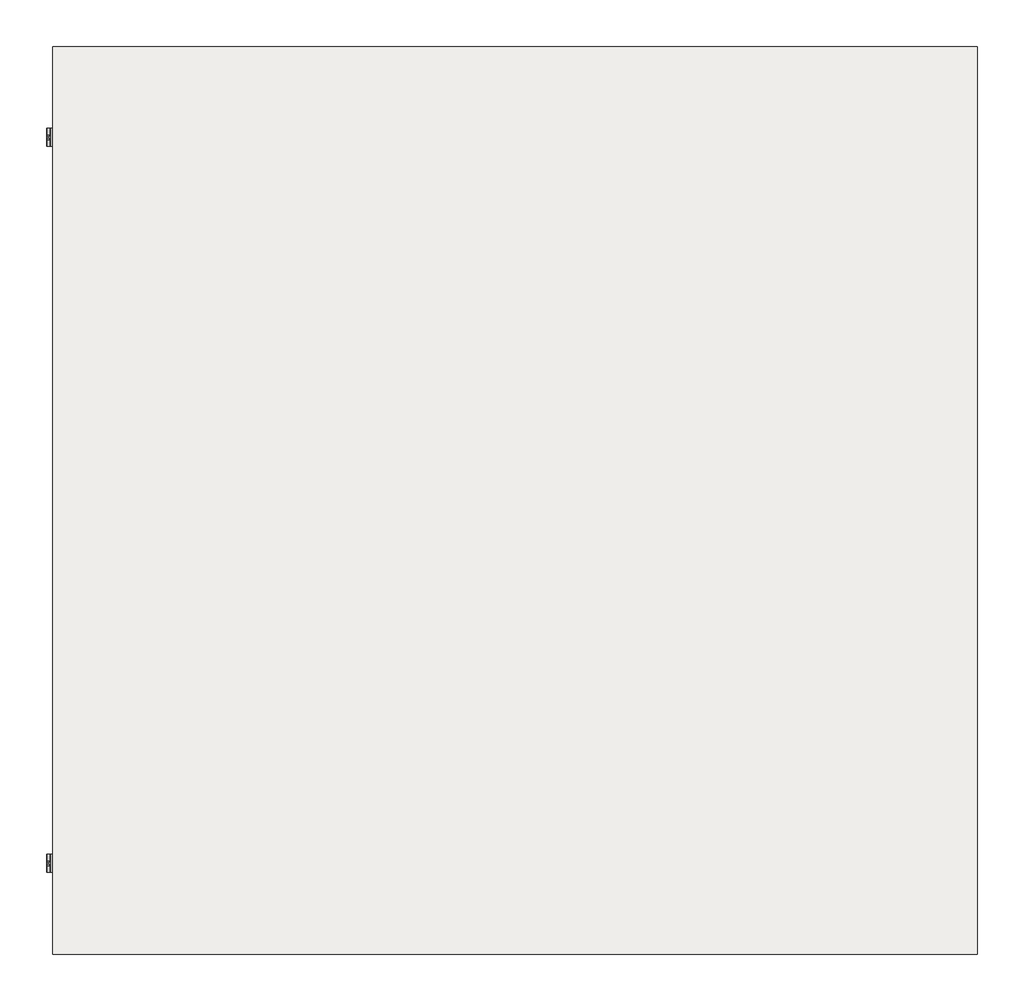
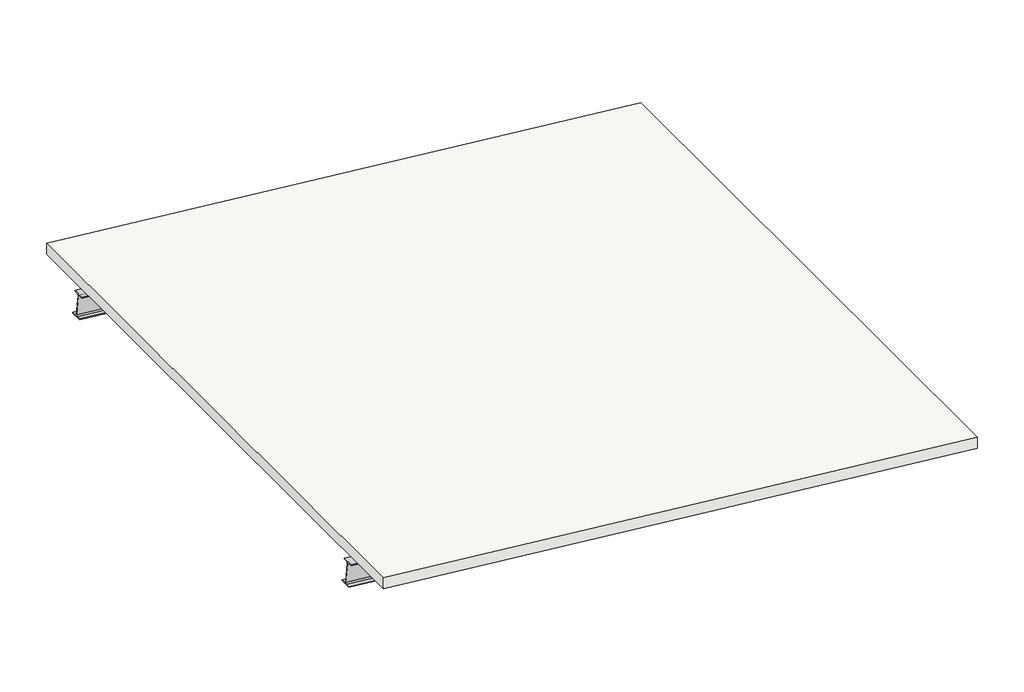
# One storey: 4 beams, 1 roof.
"""IFC4 building model written with IfcOpenShell, lengths in millimetres."""

import ifcopenshell
import ifcopenshell.guid

model = None  # the IFC model being written
_history = None  # IfcOwnerHistory: only IFC2X3 demands one
_inside = {}  # id of a spatial element -> (the spatial element, [elements in it])
_under = {}  # id of a project, library or spatial element -> (it, [spatial elements below it])
_declared = {}  # id of a project -> (the project, [libraries it declares])
_typed = {}  # id of a type object -> (the type object, [elements of that type])
_made_of = {}  # id of a material, layer set ... -> (it, [elements and type objects made of it])


def new_model(schema):
    """Start an empty IFC model of exactly this schema.

    Asked for "IFC4X3", IfcOpenShell would pick the latest addendum, in which some entities
    have other attributes; the version numbers below select the first issue.
    IFC2X3 requires an IfcOwnerHistory on every rooted entity: one is made here for all.
    """
    global model, _history
    if schema == "IFC4X3":
        model = ifcopenshell.file(schema_version=(4, 3, 0, 0))
    else:
        model = ifcopenshell.file(schema=schema)
    _inside.clear()
    _under.clear()
    _declared.clear()
    _typed.clear()
    _made_of.clear()
    _history = None
    if model.schema == "IFC2X3":
        org = make("IfcOrganization", Name="unknown")
        user = make(
            "IfcPersonAndOrganization",
            ThePerson=make("IfcPerson", FamilyName="unknown"),
            TheOrganization=org,
        )
        app = make(
            "IfcApplication",
            ApplicationDeveloper=org,
            Version="unknown",
            ApplicationFullName="unknown",
            ApplicationIdentifier="unknown",
        )
        _history = make(
            "IfcOwnerHistory",
            OwningUser=user,
            OwningApplication=app,
            ChangeAction="ADDED",
            CreationDate=0,
        )
    return model


def make(cls, **values):
    """One entity of the class cls with the attributes given. An attribute that is None is left unset."""
    return model.create_entity(
        cls, **{name: value for name, value in values.items() if value is not None}
    )


def rooted(cls, **values):
    """An entity with a GlobalId (a new one), such as an element, a storey or a relation."""
    return make(cls, GlobalId=ifcopenshell.guid.new(), OwnerHistory=_history, **values)


def si_unit(unit_type, name, prefix=None):
    """IfcSIUnit, for example si_unit("LENGTHUNIT", "METRE", prefix="MILLI")."""
    return make("IfcSIUnit", UnitType=unit_type, Prefix=prefix, Name=name)


def assignment(units):
    """IfcUnitAssignment: the units of a project."""
    return None if units is None else make("IfcUnitAssignment", Units=units)


def point(xyz):
    """IfcCartesianPoint."""
    return None if xyz is None else make("IfcCartesianPoint", Coordinates=xyz)


def direction(xyz):
    """IfcDirection."""
    return None if xyz is None else make("IfcDirection", DirectionRatios=xyz)


def frame(location, z_axis=None, x_axis=None):
    """IfcAxis2Placement3D, a coordinate frame: its origin and axes. An axis left out is left unset."""
    return make(
        "IfcAxis2Placement3D",
        Location=point(location),
        Axis=direction(z_axis),
        RefDirection=direction(x_axis),
    )


def frame_2d(location, x_axis=None):
    """IfcAxis2Placement2D, a coordinate frame in the plane: its origin and x axis."""
    return make(
        "IfcAxis2Placement2D", Location=point(location), RefDirection=direction(x_axis)
    )


def origin():
    """The frame at (0, 0, 0) with its axes left unset."""
    return frame((0.0, 0.0, 0.0))


def place(relative_to, where):
    """IfcLocalPlacement: puts the frame where relative to a parent placement (None: the world)."""
    return make(
        "IfcLocalPlacement", PlacementRelTo=relative_to, RelativePlacement=where
    )


def context(
    kind, dimensions, precision=None, world=None, true_north=None, identifier=None
):
    """IfcGeometricRepresentationContext, for example the 3D "Model" context."""
    return make(
        "IfcGeometricRepresentationContext",
        ContextIdentifier=identifier,
        ContextType=kind,
        CoordinateSpaceDimension=dimensions,
        Precision=precision,
        WorldCoordinateSystem=world,
        TrueNorth=true_north,
    )


def project(units=None, contexts=None):
    """IfcProject with its units and contexts."""
    return rooted(
        "IfcProject",
        Name="project",
        RepresentationContexts=contexts,
        UnitsInContext=assignment(units),
    )


def spatial(cls, under=None, at=None, **own):
    """A site, building, storey or space (cls), placed at a placement, below another one or the project."""
    s = rooted(cls, ObjectPlacement=at, **own)
    if under is not None:
        _under.setdefault(under.id(), (under, []))[1].append(s)
    return s


def polyline(points):
    """IfcPolyline through the points."""
    return make("IfcPolyline", Points=[point(p) for p in points])


def circle_curve(where, radius):
    """IfcCircle in the frame where."""
    return make("IfcCircle", Position=where, Radius=radius)


def trimmed(basis, trim1, trim2, sense, master):
    """IfcTrimmedCurve: the piece of a basis curve between two trims."""
    return make(
        "IfcTrimmedCurve",
        BasisCurve=basis,
        Trim1=trim1,
        Trim2=trim2,
        SenseAgreement=sense,
        MasterRepresentation=master,
    )


def segment(curve, same_sense, transition):
    """IfcCompositeCurveSegment."""
    return make(
        "IfcCompositeCurveSegment",
        Transition=transition,
        SameSense=same_sense,
        ParentCurve=curve,
    )


def composite_curve(segments, self_intersect=None):
    """IfcCompositeCurve: segments joined end to end."""
    return make("IfcCompositeCurve", Segments=segments, SelfIntersect=self_intersect)


def outline(outer, holes=None, kind="AREA"):
    """IfcArbitraryClosedProfileDef: a profile drawn as a closed curve; with holes, ...WithVoids."""
    if holes is None:
        return make("IfcArbitraryClosedProfileDef", ProfileType=kind, OuterCurve=outer)
    return make(
        "IfcArbitraryProfileDefWithVoids",
        ProfileType=kind,
        OuterCurve=outer,
        InnerCurves=holes,
    )


def extrude(swept, where, along, depth):
    """IfcExtrudedAreaSolid: the profile swept, set in the frame where, extruded along a direction by depth."""
    return make(
        "IfcExtrudedAreaSolid",
        SweptArea=swept,
        Position=where,
        ExtrudedDirection=direction(along),
        Depth=depth,
    )


def shape(context_of_items, identifier, shape_type, items):
    """IfcShapeRepresentation: the items that make up one representation, for example the "Body"."""
    return make(
        "IfcShapeRepresentation",
        ContextOfItems=context_of_items,
        RepresentationIdentifier=identifier,
        RepresentationType=shape_type,
        Items=items,
    )


def source(mapping_origin, context_of_items, identifier, shape_type, items):
    """IfcRepresentationMap: a shape defined once, which mapped items show again and again."""
    return make(
        "IfcRepresentationMap",
        MappingOrigin=mapping_origin,
        MappedRepresentation=shape(context_of_items, identifier, shape_type, items),
    )


def transform(
    local_origin,
    x_axis=None,
    y_axis=None,
    z_axis=None,
    scale=None,
    scale2=None,
    scale3=None,
    uniform=True,
):
    """IfcCartesianTransformationOperator3D, or its non-uniform kind. x_axis, y_axis, z_axis: its Axis1, 2, 3."""
    if uniform:
        return make(
            "IfcCartesianTransformationOperator3D",
            Axis1=direction(x_axis),
            Axis2=direction(y_axis),
            LocalOrigin=point(local_origin),
            Scale=scale,
            Axis3=direction(z_axis),
        )
    return make(
        "IfcCartesianTransformationOperator3DnonUniform",
        Axis1=direction(x_axis),
        Axis2=direction(y_axis),
        LocalOrigin=point(local_origin),
        Scale=scale,
        Axis3=direction(z_axis),
        Scale2=scale2,
        Scale3=scale3,
    )


def mapped(mapping_source, mapping_target):
    """IfcMappedItem: shows the shape of a source again, moved by a transform."""
    return make(
        "IfcMappedItem", MappingSource=mapping_source, MappingTarget=mapping_target
    )


def made_of(thing, what):
    """Note that an element or type object is made of a material, layer set ...; save() writes the relation."""
    if what is not None:
        _made_of.setdefault(what.id(), (what, []))[1].append(thing)
    return thing


def element(
    cls,
    number,
    at=None,
    inside=None,
    cuts=None,
    type_object=None,
    material=None,
    context=None,
    identifier="Body",
    shape_type=None,
    held_by="IfcProductDefinitionShape",
    body=None,
    shapes=None,
    **own,
):
    """One element of the class cls, such as IfcWall. Its Tag is "e" and its number.

    at: its placement. inside: the storey or other place that contains it. cuts: it is an
    opening in that element (IfcRelVoidsElement). A single representation is given by context,
    identifier, shape_type and body (its items); several are given by shapes. held_by: the class
    of the entity that holds the representations. save() writes the other relations.
    """
    e = rooted(cls, Tag="e%d" % number, ObjectPlacement=at, **own)
    if body is not None:
        shapes = [shape(context, identifier, shape_type, body)]
    if shapes is not None:
        e.Representation = make(held_by, Representations=shapes)
    if inside is not None:
        _inside.setdefault(inside.id(), (inside, []))[1].append(e)
    if cuts is not None:
        rooted(
            "IfcRelVoidsElement", RelatingBuildingElement=cuts, RelatedOpeningElement=e
        )
    if type_object is not None:
        _typed.setdefault(type_object.id(), (type_object, []))[1].append(e)
    return made_of(e, material)


def aggregate(whole, parts):
    """IfcRelAggregates: a whole, such as a stair, and the parts it consists of."""
    return rooted("IfcRelAggregates", RelatingObject=whole, RelatedObjects=parts)


def save(model, path):
    """Write the relations noted so far, then the file.

    IfcRelAggregates (storeys below a building ...), IfcRelContainedInSpatialStructure (elements
    in a storey), IfcRelDefinesByType, IfcRelAssociatesMaterial and IfcRelDeclares: one each for
    every whole, place, type object, material and project.
    """
    for whole, parts in _under.values():
        aggregate(whole, parts)
    for where, things in _inside.values():
        rooted(
            "IfcRelContainedInSpatialStructure",
            RelatedElements=things,
            RelatingStructure=where,
        )
    for kind, things in _typed.values():
        rooted("IfcRelDefinesByType", RelatedObjects=things, RelatingType=kind)
    for what, things in _made_of.values():
        rooted("IfcRelAssociatesMaterial", RelatedObjects=things, RelatingMaterial=what)
    for by, libraries in _declared.values():
        rooted("IfcRelDeclares", RelatingContext=by, RelatedDefinitions=libraries)
    model.write(path)


def beam_cef0ad3f(model_context):
    return source(origin(), model_context, "Body", "SweptSolid", [
        extrude(outline(composite_curve([segment(polyline([(50.0, -92.0), (50.0, -100.0), (-50.0, -100.0), (-50.0, -92.0), (-13.75, -92.0)]), True, "CONTINUOUS"), segment(trimmed(circle_curve(frame_2d((-13.75, -81.0)), 11.0), [point((-13.75, -92.0))], [point((-2.75, -81.0))], True, "CARTESIAN"), True, "CONTINUOUS"), segment(polyline([(-2.75, -81.0), (-2.75, 81.0)]), True, "CONTINUOUS"), segment(trimmed(circle_curve(frame_2d((-13.75, 81.0)), 11.0), [point((-2.75, 81.0))], [point((-13.75, 92.0))], True, "CARTESIAN"), True, "CONTINUOUS"), segment(polyline([(-13.75, 92.0), (-50.0, 92.0), (-50.0, 100.0), (50.0, 100.0), (50.0, 92.0), (13.75, 92.0)]), True, "CONTINUOUS"), segment(trimmed(circle_curve(frame_2d((13.75, 81.0)), 11.0), [point((13.75, 92.0))], [point((2.75, 81.0))], True, "CARTESIAN"), True, "CONTINUOUS"), segment(polyline([(2.75, 81.0), (2.75, -81.0)]), True, "CONTINUOUS"), segment(trimmed(circle_curve(frame_2d((13.75, -81.0)), 11.0), [point((2.75, -81.0))], [point((13.75, -92.0))], True, "CARTESIAN"), True, "CONTINUOUS"), segment(polyline([(13.75, -92.0), (50.0, -92.0)]), True, "CONTINUOUS")], self_intersect=False)), frame((-1887.3, 0.0, 0.0), z_axis=(1.0, 0.0, 0.0), x_axis=(0.0, 1.0, 0.0)), (0.0, 0.0, 1.0), 3774.6),
    ])


def beam_dd467f0e(model_context):
    return source(origin(), model_context, "Body", "SweptSolid", [
        extrude(outline(composite_curve([segment(polyline([(50.0, -92.0), (50.0, -100.0), (-50.0, -100.0), (-50.0, -92.0), (-13.75, -92.0)]), True, "CONTINUOUS"), segment(trimmed(circle_curve(frame_2d((-13.75, -81.0)), 11.0), [point((-13.75, -92.0))], [point((-2.75, -81.0))], True, "CARTESIAN"), True, "CONTINUOUS"), segment(polyline([(-2.75, -81.0), (-2.75, 81.0)]), True, "CONTINUOUS"), segment(trimmed(circle_curve(frame_2d((-13.75, 81.0)), 11.0), [point((-2.75, 81.0))], [point((-13.75, 92.0))], True, "CARTESIAN"), True, "CONTINUOUS"), segment(polyline([(-13.75, 92.0), (-50.0, 92.0), (-50.0, 100.0), (50.0, 100.0), (50.0, 92.0), (13.75, 92.0)]), True, "CONTINUOUS"), segment(trimmed(circle_curve(frame_2d((13.75, 81.0)), 11.0), [point((13.75, 92.0))], [point((2.75, 81.0))], True, "CARTESIAN"), True, "CONTINUOUS"), segment(polyline([(2.75, 81.0), (2.75, -81.0)]), True, "CONTINUOUS"), segment(trimmed(circle_curve(frame_2d((13.75, -81.0)), 11.0), [point((2.75, -81.0))], [point((13.75, -92.0))], True, "CARTESIAN"), True, "CONTINUOUS"), segment(polyline([(13.75, -92.0), (50.0, -92.0)]), True, "CONTINUOUS")], self_intersect=False)), frame((-2509.476368, 0.0, 0.0), z_axis=(1.0, 0.0, 0.0), x_axis=(0.0, 1.0, 0.0)), (0.0, 0.0, 1.0), 5119.4514916),
    ])


model = new_model("IFC4")

# Units and contexts
model_context = context("Model", 3, world=origin())
ifc_project = project(units=[si_unit("LENGTHUNIT", "METRE", prefix="MILLI")], contexts=[model_context])

# Site, building, storey
site = spatial("IfcSite", under=ifc_project)
building = spatial("IfcBuilding", under=site)
storey = spatial("IfcBuildingStorey", under=building, Name="TOC", Elevation=2499.9618634)

# Beams
placement = place(None, origin())
beam_shape = beam_cef0ad3f(model_context)
element("IfcBeam", 1, ObjectType="0912_Steel Framing_H-KSD3502 : H_SB_H-200x100x5.5x8", at=placement, inside=storey, context=model_context, shape_type="MappedRepresentation", body=[
    mapped(beam_shape, transform((0.0, 2499.5208589, 2799.9618634), x_axis=(0.0, 1.0, 0.0), y_axis=(-1.0, 0.0, 0.0), z_axis=(0.0, 0.0, 1.0))),
])
element("IfcBeam", 2, ObjectType="0912_Steel Framing_H-KSD3502 : H_SB_H-200x100x5.5x8", at=placement, inside=storey, context=model_context, shape_type="MappedRepresentation", body=[
    mapped(beam_shape, transform((4000.0, 2499.5208589, 2399.9618634), x_axis=(0.0, 1.0, 0.0), y_axis=(-1.0, 0.0, 0.0), z_axis=(0.0, 0.0, 1.0))),
])
beam_2_shape = beam_dd467f0e(model_context)
element("IfcBeam", 3, ObjectType="0912_Steel Framing_H-KSD3502 : H_SB_H-200x100x5.5x8", at=placement, inside=storey, context=model_context, shape_type="MappedRepresentation", body=[
    mapped(beam_2_shape, transform((2009.9503719, 499.5208589, 2799.4655824), x_axis=(0.9950371902099906, 0.0, -0.09950371902098465), y_axis=(0.0, 1.0, 0.0), z_axis=(0.09950371902098465, 0.0, 0.9950371902099906))),
])
element("IfcBeam", 4, ObjectType="0912_Steel Framing_H-KSD3502 : H_SB_H-200x100x5.5x8", at=placement, inside=storey, context=model_context, shape_type="MappedRepresentation", body=[
    mapped(beam_2_shape, transform((2009.9503719, 4499.5208589, 2799.4655824), x_axis=(0.9950371902099906, 0.0, -0.09950371902098448), y_axis=(0.0, 1.0, 0.0), z_axis=(0.09950371902098448, 0.0, 0.9950371902099906))),
])

# Roof
element("IfcRoof", 5, ObjectType="H_RF_AR_B05_Roof Panel Steel Mineral Wool T100", at=placement, inside=storey, context=model_context, shape_type="SweptSolid", body=[
    extrude(outline(polyline([(2788.5226486, 4631.8486152), (3297.9271114, -462.1960125), (3197.4283551, -462.1960125), (2688.0238924, 4631.8486152), (2788.5226486, 4631.8486152)])), frame((0.0, -0.4791411, 0.0), z_axis=(0.0, 1.0, 0.0), x_axis=(0.0, 0.0, 1.0)), (0.0, 0.0, 1.0), 5000.0),
])

save(model, "model.ifc")

# Revit data of these elements
# Type "0912_Steel Framing_H-KSD3502 : H_SB_H-200x100x5.5x8"
#   Width = 10.0 cm
#   Web Thickness = 0.55 cm
#   Web Fillet = 1.1 cm
#   Warping Constant = 12288.0 cm⁶
#   W = 0
#   Torsional Moment of Inertia = 4.4781 cm⁴
#   Section Area = 27.16 cm²
#   Plastic Modulus weak axis = 41.9 cm³
#   Plastic Modulus strong axis = 209.0 cm³
#   Perimeter = 0.77 m²/m
#   Nominal Weight = 21.30 kgf/m
#   Moment of Inertia weak axis = 134.00 cm⁴
#   Moment of Inertia strong axis = 1840.00 cm⁴
#   Height = 20.0 cm
#   Flange Thickness = 0.8 cm
#   Elastic Modulus weak axis = 26.8 cm³
#   Elastic Modulus strong axis = 184.0 cm³
#   Centroid Vertical = 10.0 cm
#   Centroid Horizontal = 5.0 cm
#   Ix = 18400000
#   Length [instance default] = 1524 mm
#   Zx = 209000
#   b = 100 mm
#   h = 200 mm
#   r = 11 mm
#   s = 5.5 mm
#   t = 8 mm
#   A = 0.002716 m²
#   Structural Material [instance default] = Steel, 45-345
#   Assembly Code = ""
# Type "H_RF_AR_B05_Roof Panel Steel Mineral Wool T100"
#   Layers, outside or top first: 100 mm no material (function 4)
# Elements 1, 2, 3, 4 (IfcBeam, "0912_Steel Framing_H-KSD3502 : H_SB_H-200x100x5.5x8")
#   Comments = ""
#   Structural Material = Steel, 45-345
#   Phase Created = New Construction
#   Materials on its faces: "Steel, 45-345"
# Element 5 (IfcRoof, "H_RF_AR_B05_Roof Panel Steel Mineral Wool T100")
#   built-in parameter 1001710 = 33615
#   Phase Created = New Construction
#   Materials on its faces: "Default Roof"
# Materials
#   "Steel, 45-345": class "Metal", colour RGB 189 187 185, transparency 0, Description = "Steel 345 MPa", Cost = 0
#   "Default Roof": class "Miscellaneous", colour RGB 80 80 80, transparency 0
